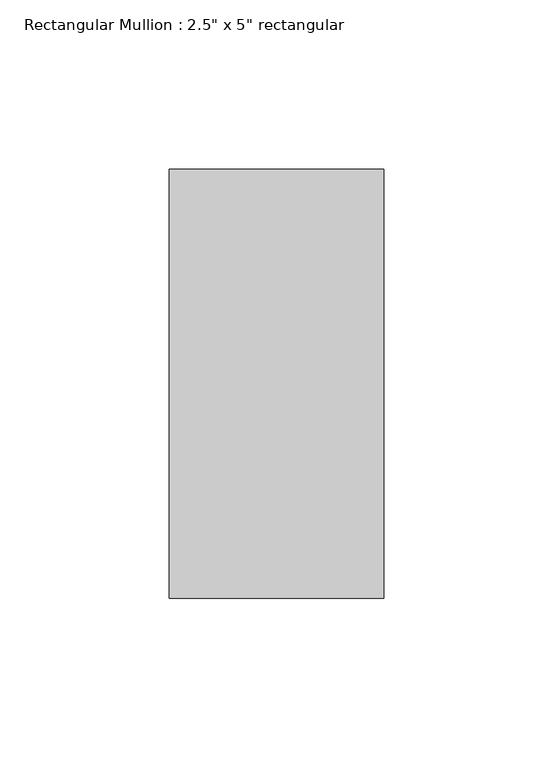
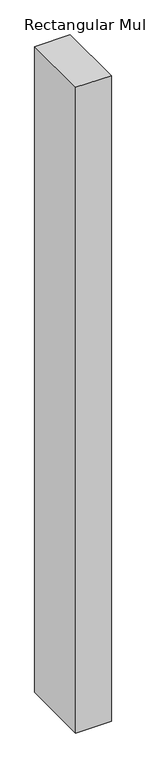
"""IFC4 building model written with IfcOpenShell, lengths in millimetres: member geometry."""

import ifcopenshell
import ifcopenshell.guid

model = None  # the IFC model being written
_history = None  # IfcOwnerHistory: only IFC2X3 demands one
_inside = {}  # id of a spatial element -> (the spatial element, [elements in it])
_under = {}  # id of a project, library or spatial element -> (it, [spatial elements below it])
_declared = {}  # id of a project -> (the project, [libraries it declares])
_typed = {}  # id of a type object -> (the type object, [elements of that type])
_made_of = {}  # id of a material, layer set ... -> (it, [elements and type objects made of it])


def new_model(schema):
    """Start an empty IFC model of exactly this schema.

    Asked for "IFC4X3", IfcOpenShell would pick the latest addendum, in which some entities
    have other attributes; the version numbers below select the first issue.
    IFC2X3 requires an IfcOwnerHistory on every rooted entity: one is made here for all.
    """
    global model, _history
    if schema == "IFC4X3":
        model = ifcopenshell.file(schema_version=(4, 3, 0, 0))
    else:
        model = ifcopenshell.file(schema=schema)
    _inside.clear()
    _under.clear()
    _declared.clear()
    _typed.clear()
    _made_of.clear()
    _history = None
    if model.schema == "IFC2X3":
        org = make("IfcOrganization", Name="unknown")
        user = make(
            "IfcPersonAndOrganization",
            ThePerson=make("IfcPerson", FamilyName="unknown"),
            TheOrganization=org,
        )
        app = make(
            "IfcApplication",
            ApplicationDeveloper=org,
            Version="unknown",
            ApplicationFullName="unknown",
            ApplicationIdentifier="unknown",
        )
        _history = make(
            "IfcOwnerHistory",
            OwningUser=user,
            OwningApplication=app,
            ChangeAction="ADDED",
            CreationDate=0,
        )
    return model


def make(cls, **values):
    """One entity of the class cls with the attributes given. An attribute that is None is left unset."""
    return model.create_entity(
        cls, **{name: value for name, value in values.items() if value is not None}
    )


def rooted(cls, **values):
    """An entity with a GlobalId (a new one), such as an element, a storey or a relation."""
    return make(cls, GlobalId=ifcopenshell.guid.new(), OwnerHistory=_history, **values)


def si_unit(unit_type, name, prefix=None):
    """IfcSIUnit, for example si_unit("LENGTHUNIT", "METRE", prefix="MILLI")."""
    return make("IfcSIUnit", UnitType=unit_type, Prefix=prefix, Name=name)


def assignment(units):
    """IfcUnitAssignment: the units of a project."""
    return None if units is None else make("IfcUnitAssignment", Units=units)


def point(xyz):
    """IfcCartesianPoint."""
    return None if xyz is None else make("IfcCartesianPoint", Coordinates=xyz)


def direction(xyz):
    """IfcDirection."""
    return None if xyz is None else make("IfcDirection", DirectionRatios=xyz)


def frame(location, z_axis=None, x_axis=None):
    """IfcAxis2Placement3D, a coordinate frame: its origin and axes. An axis left out is left unset."""
    return make(
        "IfcAxis2Placement3D",
        Location=point(location),
        Axis=direction(z_axis),
        RefDirection=direction(x_axis),
    )


def origin():
    """The frame at (0, 0, 0) with its axes left unset."""
    return frame((0.0, 0.0, 0.0))


def place(relative_to, where):
    """IfcLocalPlacement: puts the frame where relative to a parent placement (None: the world)."""
    return make(
        "IfcLocalPlacement", PlacementRelTo=relative_to, RelativePlacement=where
    )


def context(
    kind, dimensions, precision=None, world=None, true_north=None, identifier=None
):
    """IfcGeometricRepresentationContext, for example the 3D "Model" context."""
    return make(
        "IfcGeometricRepresentationContext",
        ContextIdentifier=identifier,
        ContextType=kind,
        CoordinateSpaceDimension=dimensions,
        Precision=precision,
        WorldCoordinateSystem=world,
        TrueNorth=true_north,
    )


def project(units=None, contexts=None):
    """IfcProject with its units and contexts."""
    return rooted(
        "IfcProject",
        Name="project",
        RepresentationContexts=contexts,
        UnitsInContext=assignment(units),
    )


def spatial(cls, under=None, at=None, **own):
    """A site, building, storey or space (cls), placed at a placement, below another one or the project."""
    s = rooted(cls, ObjectPlacement=at, **own)
    if under is not None:
        _under.setdefault(under.id(), (under, []))[1].append(s)
    return s


def polyline(points):
    """IfcPolyline through the points."""
    return make("IfcPolyline", Points=[point(p) for p in points])


def outline(outer, holes=None, kind="AREA"):
    """IfcArbitraryClosedProfileDef: a profile drawn as a closed curve; with holes, ...WithVoids."""
    if holes is None:
        return make("IfcArbitraryClosedProfileDef", ProfileType=kind, OuterCurve=outer)
    return make(
        "IfcArbitraryProfileDefWithVoids",
        ProfileType=kind,
        OuterCurve=outer,
        InnerCurves=holes,
    )


def extrude(swept, where, along, depth):
    """IfcExtrudedAreaSolid: the profile swept, set in the frame where, extruded along a direction by depth."""
    return make(
        "IfcExtrudedAreaSolid",
        SweptArea=swept,
        Position=where,
        ExtrudedDirection=direction(along),
        Depth=depth,
    )


def shape(context_of_items, identifier, shape_type, items):
    """IfcShapeRepresentation: the items that make up one representation, for example the "Body"."""
    return make(
        "IfcShapeRepresentation",
        ContextOfItems=context_of_items,
        RepresentationIdentifier=identifier,
        RepresentationType=shape_type,
        Items=items,
    )


def source(mapping_origin, context_of_items, identifier, shape_type, items):
    """IfcRepresentationMap: a shape defined once, which mapped items show again and again."""
    return make(
        "IfcRepresentationMap",
        MappingOrigin=mapping_origin,
        MappedRepresentation=shape(context_of_items, identifier, shape_type, items),
    )


def transform(
    local_origin,
    x_axis=None,
    y_axis=None,
    z_axis=None,
    scale=None,
    scale2=None,
    scale3=None,
    uniform=True,
):
    """IfcCartesianTransformationOperator3D, or its non-uniform kind. x_axis, y_axis, z_axis: its Axis1, 2, 3."""
    if uniform:
        return make(
            "IfcCartesianTransformationOperator3D",
            Axis1=direction(x_axis),
            Axis2=direction(y_axis),
            LocalOrigin=point(local_origin),
            Scale=scale,
            Axis3=direction(z_axis),
        )
    return make(
        "IfcCartesianTransformationOperator3DnonUniform",
        Axis1=direction(x_axis),
        Axis2=direction(y_axis),
        LocalOrigin=point(local_origin),
        Scale=scale,
        Axis3=direction(z_axis),
        Scale2=scale2,
        Scale3=scale3,
    )


def mapped(mapping_source, mapping_target):
    """IfcMappedItem: shows the shape of a source again, moved by a transform."""
    return make(
        "IfcMappedItem", MappingSource=mapping_source, MappingTarget=mapping_target
    )


def made_of(thing, what):
    """Note that an element or type object is made of a material, layer set ...; save() writes the relation."""
    if what is not None:
        _made_of.setdefault(what.id(), (what, []))[1].append(thing)
    return thing


def element(
    cls,
    number,
    at=None,
    inside=None,
    cuts=None,
    type_object=None,
    material=None,
    context=None,
    identifier="Body",
    shape_type=None,
    held_by="IfcProductDefinitionShape",
    body=None,
    shapes=None,
    **own,
):
    """One element of the class cls, such as IfcWall. Its Tag is "e" and its number.

    at: its placement. inside: the storey or other place that contains it. cuts: it is an
    opening in that element (IfcRelVoidsElement). A single representation is given by context,
    identifier, shape_type and body (its items); several are given by shapes. held_by: the class
    of the entity that holds the representations. save() writes the other relations.
    """
    e = rooted(cls, Tag="e%d" % number, ObjectPlacement=at, **own)
    if body is not None:
        shapes = [shape(context, identifier, shape_type, body)]
    if shapes is not None:
        e.Representation = make(held_by, Representations=shapes)
    if inside is not None:
        _inside.setdefault(inside.id(), (inside, []))[1].append(e)
    if cuts is not None:
        rooted(
            "IfcRelVoidsElement", RelatingBuildingElement=cuts, RelatedOpeningElement=e
        )
    if type_object is not None:
        _typed.setdefault(type_object.id(), (type_object, []))[1].append(e)
    return made_of(e, material)


def aggregate(whole, parts):
    """IfcRelAggregates: a whole, such as a stair, and the parts it consists of."""
    return rooted("IfcRelAggregates", RelatingObject=whole, RelatedObjects=parts)


def save(model, path):
    """Write the relations noted so far, then the file.

    IfcRelAggregates (storeys below a building ...), IfcRelContainedInSpatialStructure (elements
    in a storey), IfcRelDefinesByType, IfcRelAssociatesMaterial and IfcRelDeclares: one each for
    every whole, place, type object, material and project.
    """
    for whole, parts in _under.values():
        aggregate(whole, parts)
    for where, things in _inside.values():
        rooted(
            "IfcRelContainedInSpatialStructure",
            RelatedElements=things,
            RelatingStructure=where,
        )
    for kind, things in _typed.values():
        rooted("IfcRelDefinesByType", RelatedObjects=things, RelatingType=kind)
    for what, things in _made_of.values():
        rooted("IfcRelAssociatesMaterial", RelatedObjects=things, RelatingMaterial=what)
    for by, libraries in _declared.values():
        rooted("IfcRelDeclares", RelatingContext=by, RelatedDefinitions=libraries)
    model.write(path)


def member_2b49869a(model_context):
    return source(origin(), model_context, "Body", "SweptSolid", [
        extrude(outline(polyline([(31.75, 63.5), (31.75, -63.5), (-31.75, -63.5), (-31.75, 63.5), (31.75, 63.5)])), frame((0.0, 0.0, -1219.2), z_axis=(0.0, 0.0, 1.0), x_axis=(1.0, 0.0, 0.0)), (0.0, 0.0, 1.0), 1219.2),
    ])


if __name__ == "__main__":
    model = new_model("IFC4")
    model_context = context("Model", 3, world=origin())
    ifc_project = project(units=[si_unit("LENGTHUNIT", "METRE", prefix="MILLI")], contexts=[model_context])
    site = spatial("IfcSite", under=ifc_project)
    building = spatial("IfcBuilding", under=site)
    placement = place(None, origin())
    member_shape = member_2b49869a(model_context)
    element("IfcMember", 1, ObjectType="Rectangular Mullion : 2.5\" x 5\" rectangular", at=placement, inside=building, context=model_context, shape_type="MappedRepresentation", body=[
        mapped(member_shape, transform((0.0, 0.0, 0.0), x_axis=(1.0, 0.0, 0.0), y_axis=(0.0, 1.0, 0.0), z_axis=(0.0, 0.0, 1.0))),
    ])
    save(model, "model.ifc")

# Revit data of these elements
# Type "Rectangular Mullion : 2.5\" x 5\" rectangular"
#   built-in parameter 1007304 = 0.416667 (stored number, unit not read)
#   built-in parameter 1007301 = 0.104167 (stored number, unit not read)
#   built-in parameter 1007300 = 0.104167 (stored number, unit not read)
# Element 1 (IfcMember, "Rectangular Mullion : 2.5\" x 5\" rectangular")
#   Materials on its faces: "Aluminum"
# Materials
#   "Aluminum": class "Metal", colour RGB 247 247 247, transparency 0, Description = "Aluminum 6061", Cost = 0
